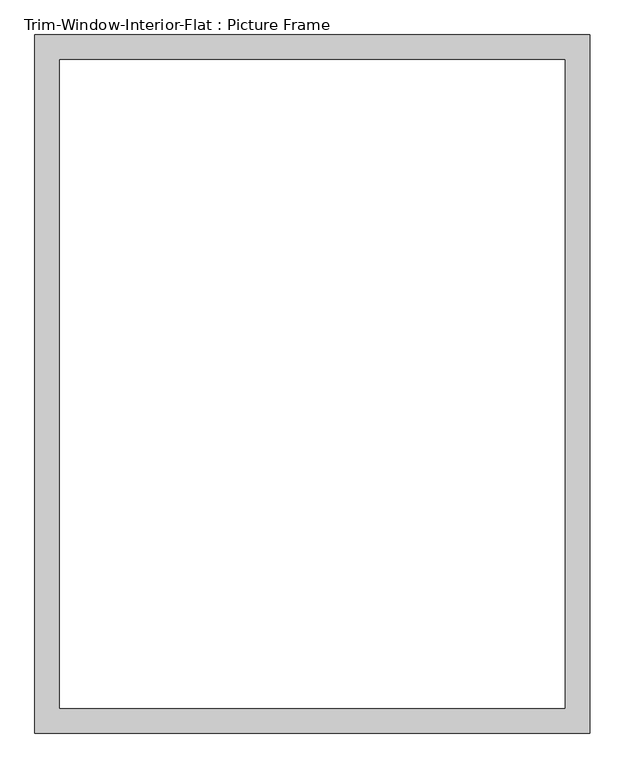
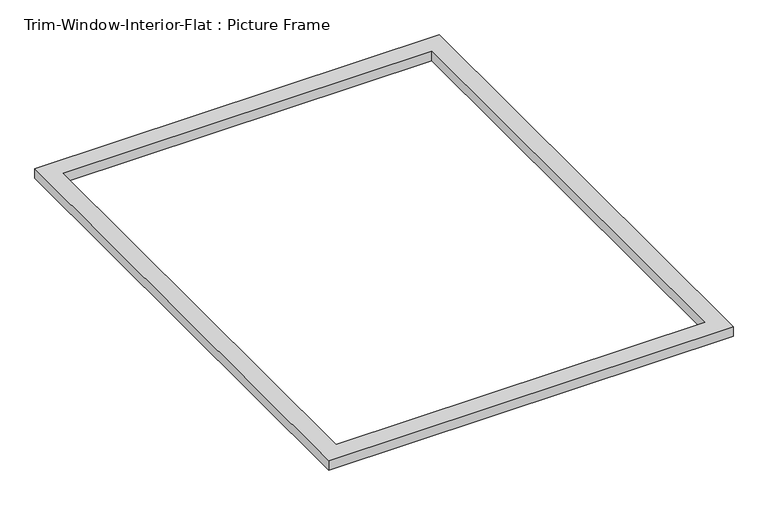
"""IFC4 building model written with IfcOpenShell, lengths in millimetres: proxy geometry, Trim-Window-Interior-Flat : Picture Frame."""

import ifcopenshell
import ifcopenshell.guid

model = None  # the IFC model being written
_history = None  # IfcOwnerHistory: only IFC2X3 demands one
_inside = {}  # id of a spatial element -> (the spatial element, [elements in it])
_under = {}  # id of a project, library or spatial element -> (it, [spatial elements below it])
_declared = {}  # id of a project -> (the project, [libraries it declares])
_typed = {}  # id of a type object -> (the type object, [elements of that type])
_made_of = {}  # id of a material, layer set ... -> (it, [elements and type objects made of it])


def new_model(schema):
    """Start an empty IFC model of exactly this schema.

    Asked for "IFC4X3", IfcOpenShell would pick the latest addendum, in which some entities
    have other attributes; the version numbers below select the first issue.
    IFC2X3 requires an IfcOwnerHistory on every rooted entity: one is made here for all.
    """
    global model, _history
    if schema == "IFC4X3":
        model = ifcopenshell.file(schema_version=(4, 3, 0, 0))
    else:
        model = ifcopenshell.file(schema=schema)
    _inside.clear()
    _under.clear()
    _declared.clear()
    _typed.clear()
    _made_of.clear()
    _history = None
    if model.schema == "IFC2X3":
        org = make("IfcOrganization", Name="unknown")
        user = make(
            "IfcPersonAndOrganization",
            ThePerson=make("IfcPerson", FamilyName="unknown"),
            TheOrganization=org,
        )
        app = make(
            "IfcApplication",
            ApplicationDeveloper=org,
            Version="unknown",
            ApplicationFullName="unknown",
            ApplicationIdentifier="unknown",
        )
        _history = make(
            "IfcOwnerHistory",
            OwningUser=user,
            OwningApplication=app,
            ChangeAction="ADDED",
            CreationDate=0,
        )
    return model


def make(cls, **values):
    """One entity of the class cls with the attributes given. An attribute that is None is left unset."""
    return model.create_entity(
        cls, **{name: value for name, value in values.items() if value is not None}
    )


def rooted(cls, **values):
    """An entity with a GlobalId (a new one), such as an element, a storey or a relation."""
    return make(cls, GlobalId=ifcopenshell.guid.new(), OwnerHistory=_history, **values)


def si_unit(unit_type, name, prefix=None):
    """IfcSIUnit, for example si_unit("LENGTHUNIT", "METRE", prefix="MILLI")."""
    return make("IfcSIUnit", UnitType=unit_type, Prefix=prefix, Name=name)


def assignment(units):
    """IfcUnitAssignment: the units of a project."""
    return None if units is None else make("IfcUnitAssignment", Units=units)


def point(xyz):
    """IfcCartesianPoint."""
    return None if xyz is None else make("IfcCartesianPoint", Coordinates=xyz)


def direction(xyz):
    """IfcDirection."""
    return None if xyz is None else make("IfcDirection", DirectionRatios=xyz)


def frame(location, z_axis=None, x_axis=None):
    """IfcAxis2Placement3D, a coordinate frame: its origin and axes. An axis left out is left unset."""
    return make(
        "IfcAxis2Placement3D",
        Location=point(location),
        Axis=direction(z_axis),
        RefDirection=direction(x_axis),
    )


def origin():
    """The frame at (0, 0, 0) with its axes left unset."""
    return frame((0.0, 0.0, 0.0))


def origin_with_axes():
    """The frame at (0, 0, 0) with the z axis (0, 0, 1) and the x axis (1, 0, 0) written out."""
    return frame((0.0, 0.0, 0.0), z_axis=(0.0, 0.0, 1.0), x_axis=(1.0, 0.0, 0.0))


def place(relative_to, where):
    """IfcLocalPlacement: puts the frame where relative to a parent placement (None: the world)."""
    return make(
        "IfcLocalPlacement", PlacementRelTo=relative_to, RelativePlacement=where
    )


def context(
    kind, dimensions, precision=None, world=None, true_north=None, identifier=None
):
    """IfcGeometricRepresentationContext, for example the 3D "Model" context."""
    return make(
        "IfcGeometricRepresentationContext",
        ContextIdentifier=identifier,
        ContextType=kind,
        CoordinateSpaceDimension=dimensions,
        Precision=precision,
        WorldCoordinateSystem=world,
        TrueNorth=true_north,
    )


def project(units=None, contexts=None):
    """IfcProject with its units and contexts."""
    return rooted(
        "IfcProject",
        Name="project",
        RepresentationContexts=contexts,
        UnitsInContext=assignment(units),
    )


def spatial(cls, under=None, at=None, **own):
    """A site, building, storey or space (cls), placed at a placement, below another one or the project."""
    s = rooted(cls, ObjectPlacement=at, **own)
    if under is not None:
        _under.setdefault(under.id(), (under, []))[1].append(s)
    return s


def polyline(points):
    """IfcPolyline through the points."""
    return make("IfcPolyline", Points=[point(p) for p in points])


def outline(outer, holes=None, kind="AREA"):
    """IfcArbitraryClosedProfileDef: a profile drawn as a closed curve; with holes, ...WithVoids."""
    if holes is None:
        return make("IfcArbitraryClosedProfileDef", ProfileType=kind, OuterCurve=outer)
    return make(
        "IfcArbitraryProfileDefWithVoids",
        ProfileType=kind,
        OuterCurve=outer,
        InnerCurves=holes,
    )


def extrude(swept, where, along, depth):
    """IfcExtrudedAreaSolid: the profile swept, set in the frame where, extruded along a direction by depth."""
    return make(
        "IfcExtrudedAreaSolid",
        SweptArea=swept,
        Position=where,
        ExtrudedDirection=direction(along),
        Depth=depth,
    )


def shape(context_of_items, identifier, shape_type, items):
    """IfcShapeRepresentation: the items that make up one representation, for example the "Body"."""
    return make(
        "IfcShapeRepresentation",
        ContextOfItems=context_of_items,
        RepresentationIdentifier=identifier,
        RepresentationType=shape_type,
        Items=items,
    )


def source(mapping_origin, context_of_items, identifier, shape_type, items):
    """IfcRepresentationMap: a shape defined once, which mapped items show again and again."""
    return make(
        "IfcRepresentationMap",
        MappingOrigin=mapping_origin,
        MappedRepresentation=shape(context_of_items, identifier, shape_type, items),
    )


def transform(
    local_origin,
    x_axis=None,
    y_axis=None,
    z_axis=None,
    scale=None,
    scale2=None,
    scale3=None,
    uniform=True,
):
    """IfcCartesianTransformationOperator3D, or its non-uniform kind. x_axis, y_axis, z_axis: its Axis1, 2, 3."""
    if uniform:
        return make(
            "IfcCartesianTransformationOperator3D",
            Axis1=direction(x_axis),
            Axis2=direction(y_axis),
            LocalOrigin=point(local_origin),
            Scale=scale,
            Axis3=direction(z_axis),
        )
    return make(
        "IfcCartesianTransformationOperator3DnonUniform",
        Axis1=direction(x_axis),
        Axis2=direction(y_axis),
        LocalOrigin=point(local_origin),
        Scale=scale,
        Axis3=direction(z_axis),
        Scale2=scale2,
        Scale3=scale3,
    )


def mapped(mapping_source, mapping_target):
    """IfcMappedItem: shows the shape of a source again, moved by a transform."""
    return make(
        "IfcMappedItem", MappingSource=mapping_source, MappingTarget=mapping_target
    )


def made_of(thing, what):
    """Note that an element or type object is made of a material, layer set ...; save() writes the relation."""
    if what is not None:
        _made_of.setdefault(what.id(), (what, []))[1].append(thing)
    return thing


def element(
    cls,
    number,
    at=None,
    inside=None,
    cuts=None,
    type_object=None,
    material=None,
    context=None,
    identifier="Body",
    shape_type=None,
    held_by="IfcProductDefinitionShape",
    body=None,
    shapes=None,
    **own,
):
    """One element of the class cls, such as IfcWall. Its Tag is "e" and its number.

    at: its placement. inside: the storey or other place that contains it. cuts: it is an
    opening in that element (IfcRelVoidsElement). A single representation is given by context,
    identifier, shape_type and body (its items); several are given by shapes. held_by: the class
    of the entity that holds the representations. save() writes the other relations.
    """
    e = rooted(cls, Tag="e%d" % number, ObjectPlacement=at, **own)
    if body is not None:
        shapes = [shape(context, identifier, shape_type, body)]
    if shapes is not None:
        e.Representation = make(held_by, Representations=shapes)
    if inside is not None:
        _inside.setdefault(inside.id(), (inside, []))[1].append(e)
    if cuts is not None:
        rooted(
            "IfcRelVoidsElement", RelatingBuildingElement=cuts, RelatedOpeningElement=e
        )
    if type_object is not None:
        _typed.setdefault(type_object.id(), (type_object, []))[1].append(e)
    return made_of(e, material)


def aggregate(whole, parts):
    """IfcRelAggregates: a whole, such as a stair, and the parts it consists of."""
    return rooted("IfcRelAggregates", RelatingObject=whole, RelatedObjects=parts)


def save(model, path):
    """Write the relations noted so far, then the file.

    IfcRelAggregates (storeys below a building ...), IfcRelContainedInSpatialStructure (elements
    in a storey), IfcRelDefinesByType, IfcRelAssociatesMaterial and IfcRelDeclares: one each for
    every whole, place, type object, material and project.
    """
    for whole, parts in _under.values():
        aggregate(whole, parts)
    for where, things in _inside.values():
        rooted(
            "IfcRelContainedInSpatialStructure",
            RelatedElements=things,
            RelatingStructure=where,
        )
    for kind, things in _typed.values():
        rooted("IfcRelDefinesByType", RelatedObjects=things, RelatingType=kind)
    for what, things in _made_of.values():
        rooted("IfcRelAssociatesMaterial", RelatedObjects=things, RelatingMaterial=what)
    for by, libraries in _declared.values():
        rooted("IfcRelDeclares", RelatingContext=by, RelatedDefinitions=libraries)
    model.write(path)


def trim_window_interior_flat_picture_frame_d5efd988(model_context):
    return source(origin(), model_context, "Body", "SweptSolid", [
        extrude(outline(polyline([(641.35, 44.45), (641.35, -1568.45), (-641.35, -1568.45), (-641.35, 44.45), (641.35, 44.45)]), holes=[polyline([(584.2, -12.7), (-584.2, -12.7), (-584.2, -1511.3), (584.2, -1511.3), (584.2, -12.7)])]), origin_with_axes(), (0.0, 0.0, 1.0), 31.75),
    ])


if __name__ == "__main__":
    model = new_model("IFC4")
    model_context = context("Model", 3, world=origin())
    ifc_project = project(units=[si_unit("LENGTHUNIT", "METRE", prefix="MILLI")], contexts=[model_context])
    site = spatial("IfcSite", under=ifc_project)
    building = spatial("IfcBuilding", under=site)
    placement = place(None, origin())
    trim_window_interior_flat_picture_frame_shape = trim_window_interior_flat_picture_frame_d5efd988(model_context)
    element("IfcBuildingElementProxy", 1, Name="Trim-Window-Interior-Flat : Picture Frame", ObjectType="Trim-Window-Interior-Flat : Picture Frame", at=placement, inside=building, context=model_context, shape_type="MappedRepresentation", body=[
        mapped(trim_window_interior_flat_picture_frame_shape, transform((0.0, 0.0, 0.0), x_axis=(1.0, 0.0, 0.0), y_axis=(0.0, 1.0, 0.0), z_axis=(0.0, 0.0, 1.0))),
    ])
    save(model, "model.ifc")

# Revit data of these elements
# Type "Trim-Window-Interior-Flat : Picture Frame"
#   Trim Thickness_Picture Frame = 0' - 1 1/4"
#   Trim Width = 0' - 2 1/4"
#   Trim Thickness_with Sill = 0' - 0 3/4"
#   Sill Thickness = 0' - 1 1/4"
#   Opening Width [instance default] = 2' - 0"
#   Opening Height [instance default] = 3' - 0"
#   Default Elevation = 4' - 0"
#   Sill = no
#   Picture Frame = yes
#   Trim Material [instance default] = none
# Element 1 (IfcBuildingElementProxy, "Trim-Window-Interior-Flat : Picture Frame")
#   Opening Width = 3' - 11"
#   Opening Height = 5' - 0"
#   Trim Material = Wood - Stained
#   Materials on its faces: "Wood - Stained"
# Materials
#   "Wood - Stained": class "Wood", colour RGB 224 178 126, transparency 0, Cost = 0
